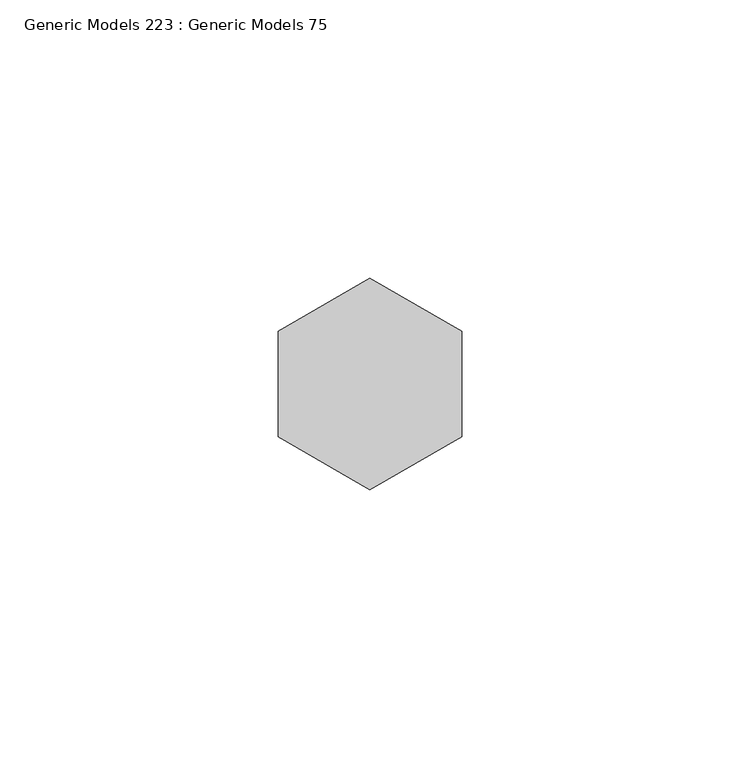
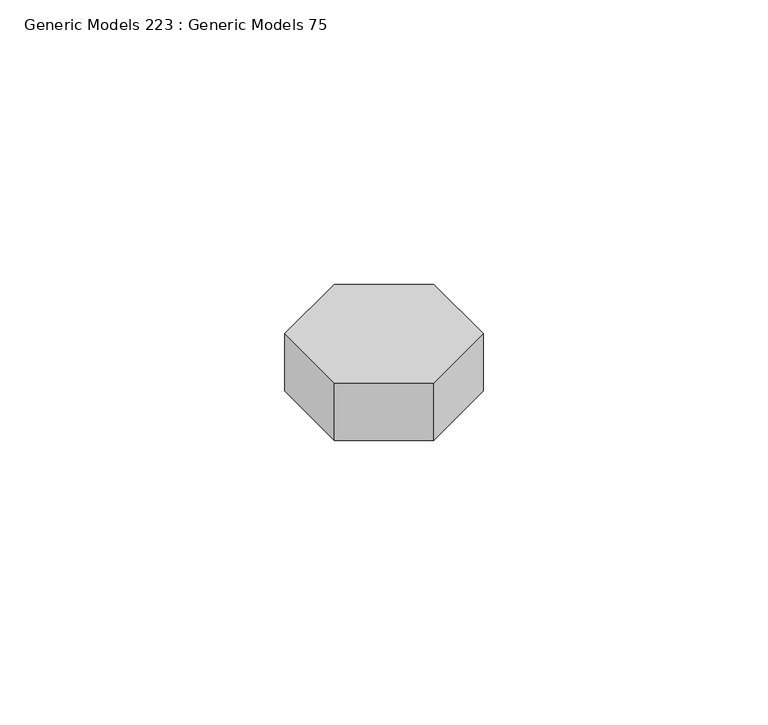
"""IFC4 building model written with IfcOpenShell, lengths in millimetres: proxy geometry, Generic Models 223 : Generic Models 75."""

from ifc_helpers import new_model, si_unit, frame, origin, place, context, project, spatial, polyline, outline, extrude, source, transform, mapped, element, save


def generic_models_223_generic_models_75_094c897c(model_context):
    return source(origin(), model_context, "Body", "SweptSolid", [
        extrude(outline(polyline([(32004.6193618, 30887.1007369), (31988.1215778, 30877.5757369), (31971.6237939, 30887.1007369), (31971.6237939, 30906.1507369), (31988.1215778, 30915.6757369), (32004.6193618, 30906.1507369), (32004.6193618, 30887.1007369)])), frame((0.0, 0.0, 266422.1875), z_axis=(0.0, 0.0, 1.0), x_axis=(1.0, 0.0, 0.0)), (0.0, 0.0, 1.0), 13.49375),
    ])


if __name__ == "__main__":
    model = new_model("IFC4")
    model_context = context("Model", 3, world=origin())
    ifc_project = project(units=[si_unit("LENGTHUNIT", "METRE", prefix="MILLI")], contexts=[model_context])
    site = spatial("IfcSite", under=ifc_project)
    building = spatial("IfcBuilding", under=site)
    placement = place(None, origin())
    generic_models_223_generic_models_75_shape = generic_models_223_generic_models_75_094c897c(model_context)
    element("IfcBuildingElementProxy", 1, Name="Generic Models 223 : Generic Models 75", ObjectType="Generic Models 223 : Generic Models 75", at=placement, inside=building, context=model_context, shape_type="MappedRepresentation", body=[
        mapped(generic_models_223_generic_models_75_shape, transform((0.0, 0.0, 0.0), x_axis=(1.0, 0.0, 0.0), y_axis=(0.0, 1.0, 0.0), z_axis=(0.0, 0.0, 1.0))),
    ])
    save(model, "model.ifc")

# Revit data of these elements
# Element 1 (IfcBuildingElementProxy, "Generic Models 223 : Generic Models 75")
#   Materials on its faces: "5/8\" DIA. EPOXY ANCHOR BOLTS"
# Materials
#   "5/8\" DIA. EPOXY ANCHOR BOLTS": class "Metal", colour RGB 199 199 199, transparency 0, Description = "Carbon steel", Cost = 0
